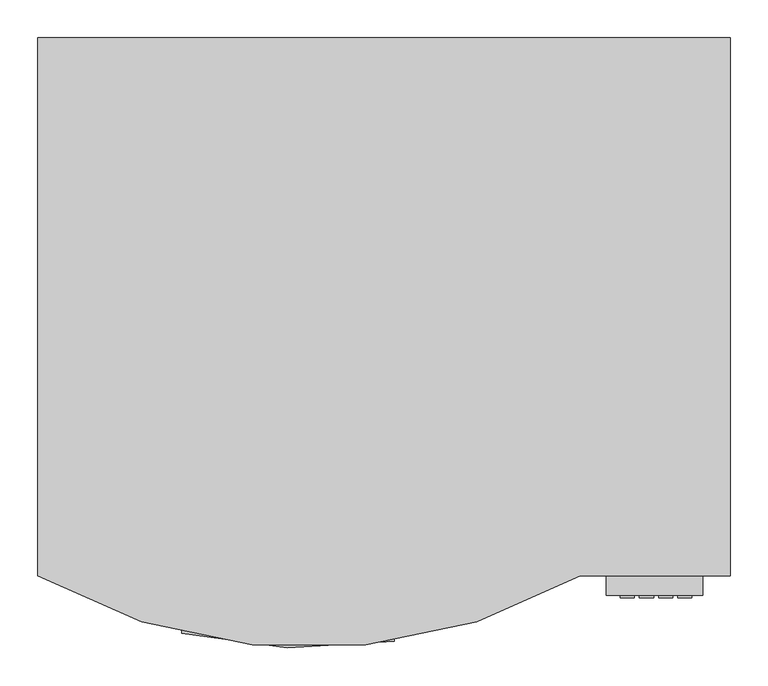
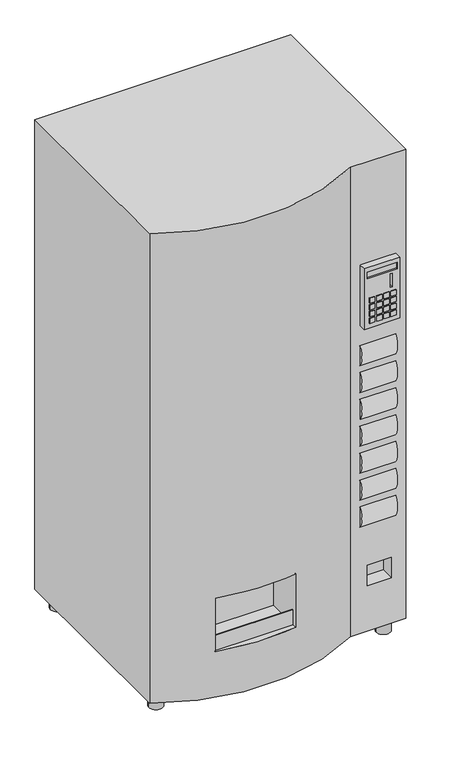
"""IFC4 building model written with IfcOpenShell, lengths in millimetres: proxy geometry, Getränkeautomat : Getränkeautomat."""

from ifc_helpers import new_model, si_unit, point, frame, frame_2d, origin, origin_with_axes, place, context, project, spatial, polyline, circle_curve, trimmed, segment, composite_curve, outline, extrude, faceted_brep, source, transform, mapped, element, save
from ifc_brep_helpers import plane_surface, cylinder_surface, advanced_brep


def specialty_equipment_d6c7ff97(model_context):
    return source(origin(), model_context, "Body", "SolidModel", [
        extrude(outline(composite_curve([segment(trimmed(circle_curve(frame_2d((-216.0902216, 1105.4279487)), 67.5221597), [point((-271.8363609, 1067.3279487))], [point((-271.8363609, 1143.5279487))], False, "CARTESIAN"), True, "CONTINUOUS"), segment(polyline([(-271.8363609, 1143.5279487), (-271.8363609, 1067.3279487)]), True, "CONTINUOUS")], self_intersect=False)), frame((275.3159229, 0.0, 0.0), z_axis=(1.0, 0.0, 0.0), x_axis=(0.0, 1.0, 0.0)), (0.0, 0.0, 1.0), 127.0948963),
        extrude(outline(composite_curve([segment(trimmed(circle_curve(frame_2d((-216.0902216, 1003.8279487)), 67.5221597), [point((-271.8363609, 965.7279487))], [point((-271.8363609, 1041.9279487))], False, "CARTESIAN"), True, "CONTINUOUS"), segment(polyline([(-271.8363609, 1041.9279487), (-271.8363609, 965.7279487)]), True, "CONTINUOUS")], self_intersect=False)), frame((275.3159229, 0.0, 0.0), z_axis=(1.0, 0.0, 0.0), x_axis=(0.0, 1.0, 0.0)), (0.0, 0.0, 1.0), 127.0948963),
        extrude(outline(composite_curve([segment(trimmed(circle_curve(frame_2d((-216.0902216, 902.2279487)), 67.5221597), [point((-271.8363609, 864.1279487))], [point((-271.8363609, 940.3279487))], False, "CARTESIAN"), True, "CONTINUOUS"), segment(polyline([(-271.8363609, 940.3279487), (-271.8363609, 864.1279487)]), True, "CONTINUOUS")], self_intersect=False)), frame((275.3159229, 0.0, 0.0), z_axis=(1.0, 0.0, 0.0), x_axis=(0.0, 1.0, 0.0)), (0.0, 0.0, 1.0), 127.0948963),
        extrude(outline(composite_curve([segment(trimmed(circle_curve(frame_2d((-216.0902216, 800.6279487)), 67.5221597), [point((-271.8363609, 762.5279487))], [point((-271.8363609, 838.7279487))], False, "CARTESIAN"), True, "CONTINUOUS"), segment(polyline([(-271.8363609, 838.7279487), (-271.8363609, 762.5279487)]), True, "CONTINUOUS")], self_intersect=False)), frame((275.3159229, 0.0, 0.0), z_axis=(1.0, 0.0, 0.0), x_axis=(0.0, 1.0, 0.0)), (0.0, 0.0, 1.0), 127.0948963),
        extrude(outline(composite_curve([segment(trimmed(circle_curve(frame_2d((-216.0902216, 699.0279487)), 67.5221597), [point((-271.8363609, 660.9279487))], [point((-271.8363609, 737.1279487))], False, "CARTESIAN"), True, "CONTINUOUS"), segment(polyline([(-271.8363609, 737.1279487), (-271.8363609, 660.9279487)]), True, "CONTINUOUS")], self_intersect=False)), frame((275.3159229, 0.0, 0.0), z_axis=(1.0, 0.0, 0.0), x_axis=(0.0, 1.0, 0.0)), (0.0, 0.0, 1.0), 127.0948963),
        extrude(outline(composite_curve([segment(trimmed(circle_curve(frame_2d((-216.0902216, 597.4279487)), 67.5221597), [point((-271.8363609, 559.3279487))], [point((-271.8363609, 635.5279487))], False, "CARTESIAN"), True, "CONTINUOUS"), segment(polyline([(-271.8363609, 635.5279487), (-271.8363609, 559.3279487)]), True, "CONTINUOUS")], self_intersect=False)), frame((275.3159229, 0.0, 0.0), z_axis=(1.0, 0.0, 0.0), x_axis=(0.0, 1.0, 0.0)), (0.0, 0.0, 1.0), 127.0948963),
        extrude(outline(composite_curve([segment(trimmed(circle_curve(frame_2d((-216.0902216, 495.8279487)), 67.5221597), [point((-271.8363609, 457.7279487))], [point((-271.8363609, 533.9279487))], False, "CARTESIAN"), True, "CONTINUOUS"), segment(polyline([(-271.8363609, 533.9279487), (-271.8363609, 457.7279487)]), True, "CONTINUOUS")], self_intersect=False)), frame((275.3159229, 0.0, 0.0), z_axis=(1.0, 0.0, 0.0), x_axis=(0.0, 1.0, 0.0)), (0.0, 0.0, 1.0), 127.0948963),
        faceted_brep([(402.3159229, -297.2363609, 1448.3279487), (275.3159229, -297.2363609, 1448.3279487), (275.3159229, -297.2363609, 1219.7279487), (402.3159229, -297.2363609, 1219.7279487), (286.3445758, -297.2363609, 1432.5207795), (394.2945758, -297.2363609, 1432.5207795), (394.2945758, -297.2363609, 1407.1207795), (286.3445758, -297.2363609, 1407.1207795), (369.009172, -297.2363609, 1397.7730022), (375.359172, -297.2363609, 1397.7730022), (375.359172, -297.2363609, 1346.9730022), (369.009172, -297.2363609, 1346.9730022), (402.3159229, -271.8363609, 1448.3279487), (402.3159229, -271.8363609, 1219.7279487), (275.3159229, -271.8363609, 1219.7279487), (275.3159229, -271.8363609, 1448.3279487), (394.2945758, -290.8863609, 1432.5207795), (286.3445758, -290.8863609, 1432.5207795), (286.3445758, -290.8863609, 1407.1207795), (394.2945758, -290.8863609, 1407.1207795), (375.359172, -275.0113609, 1397.7730022), (369.009172, -275.0113609, 1397.7730022), (369.009172, -275.0113609, 1346.9730022), (375.359172, -275.0113609, 1346.9730022)], [[[0, 1, 2, 3], [4, 5, 6, 7], [8, 9, 10, 11]], [[12, 13, 14, 15]], [[1, 0, 12, 15]], [[2, 1, 15, 14]], [[3, 2, 14, 13]], [[0, 3, 13, 12]], [[16, 17, 18, 19]], [[17, 16, 5, 4]], [[18, 17, 4, 7]], [[19, 18, 7, 6]], [[16, 19, 6, 5]], [[20, 21, 22, 23]], [[21, 20, 9, 8]], [[22, 21, 8, 11]], [[23, 22, 11, 10]], [[20, 23, 10, 9]]]),
        extrude(outline(polyline([(-4.9505365, -342.4801109), (-285.8560243, -342.4801109), (-285.8560243, -339.3678837), (-4.9505365, -339.3678837), (-4.9505365, -342.4801109)])), frame((0.0, 0.0, 227.0552601), z_axis=(0.0, 0.0, 1.0), x_axis=(1.0, 0.0, 0.0)), (0.0, 0.0, 1.0), 59.7862005),
        extrude(outline(composite_curve([segment(trimmed(circle_curve(frame_2d((-424.8751183, 388.5636391)), 25.4), [point((-450.2751183, 388.5636391))], [point((-399.4751183, 388.5636391))], False, "CARTESIAN"), True, "CONTINUOUS"), segment(trimmed(circle_curve(frame_2d((-424.8751183, 388.5636391)), 25.4), [point((-399.4751183, 388.5636391))], [point((-450.2751183, 388.5636391))], False, "CARTESIAN"), True, "CONTINUOUS")], self_intersect=False)), origin_with_axes(), (0.0, 0.0, 1.0), 55.5625),
        extrude(outline(composite_curve([segment(trimmed(circle_curve(frame_2d((387.9248817, 388.5636391)), 25.4), [point((362.5248817, 388.5636391))], [point((413.3248817, 388.5636391))], False, "CARTESIAN"), True, "CONTINUOUS"), segment(trimmed(circle_curve(frame_2d((387.9248817, 388.5636391)), 25.4), [point((413.3248817, 388.5636391))], [point((362.5248817, 388.5636391))], False, "CARTESIAN"), True, "CONTINUOUS")], self_intersect=False)), origin_with_axes(), (0.0, 0.0, 1.0), 55.5625),
        extrude(outline(composite_curve([segment(trimmed(circle_curve(frame_2d((387.9248817, -221.0363609)), 25.4), [point((362.5248817, -221.0363609))], [point((413.3248817, -221.0363609))], False, "CARTESIAN"), True, "CONTINUOUS"), segment(trimmed(circle_curve(frame_2d((387.9248817, -221.0363609)), 25.4), [point((413.3248817, -221.0363609))], [point((362.5248817, -221.0363609))], False, "CARTESIAN"), True, "CONTINUOUS")], self_intersect=False)), origin_with_axes(), (0.0, 0.0, 1.0), 55.5625),
        extrude(outline(composite_curve([segment(trimmed(circle_curve(frame_2d((-424.8751183, -221.0363609)), 25.4), [point((-450.2751183, -221.0363609))], [point((-399.4751183, -221.0363609))], False, "CARTESIAN"), True, "CONTINUOUS"), segment(trimmed(circle_curve(frame_2d((-424.8751183, -221.0363609)), 25.4), [point((-399.4751183, -221.0363609))], [point((-450.2751183, -221.0363609))], False, "CARTESIAN"), True, "CONTINUOUS")], self_intersect=False)), origin_with_axes(), (0.0, 0.0, 1.0), 55.5625),
        advanced_brep(
        [(438.7248817, 439.3636391, 1828.8), (-475.6751183, 439.3636391, 1828.8), (-475.6751183, -271.8363609, 1828.8), (240.962407, -271.8363609, 1828.8), (438.7248817, -271.8363609, 1828.8), (438.7248817, 439.3636391, 55.4895962), (438.7248817, -271.8363609, 55.4895962), (240.962407, -271.8363609, 55.4895962), (-475.6751183, -271.8363609, 55.4895962), (-475.6751183, 439.3636391, 55.4895962), (-285.8560243, -347.1225541, 431.8), (-4.9505365, -358.2607189, 431.8), (-4.9505365, -358.2607189, 229.9895559), (-285.8560243, -347.1225541, 229.9895559), (387.9248817, -271.8363609, 304.8), (387.9248817, -271.8363609, 227.0552601), (301.300731, -271.8363609, 227.0552601), (301.300731, -271.8363609, 304.8), (-4.9505365, -221.0363609, 431.8), (-285.8560243, -221.0363609, 431.8), (-285.8560243, -221.0363609, 229.9895559), (-4.9505365, -221.0363609, 229.9895559), (387.9248817, -221.0363609, 304.8), (301.300731, -221.0363609, 304.8), (301.300731, -221.0363609, 227.0552601), (387.9248817, -221.0363609, 227.0552601)],
        [
            (0, 1),
            (1, 2),
            (2, 3, circle_curve(frame((-117.3563557, 354.6542517, 1828.8), z_axis=(0.0, 0.0, 1.0), x_axis=(1.0, 0.0, 0.0)), 721.7221234)),
            (3, 4),
            (4, 0),
            (5, 6),
            (6, 7),
            (7, 8, circle_curve(frame((-117.3563557, 354.6542517, 55.4895962), z_axis=(0.0, 0.0, -1.0), x_axis=(1.0, 0.0, 0.0)), 721.7221234)),
            (8, 9),
            (9, 5),
            (0, 5),
            (9, 1),
            (8, 2),
            (7, 3),
            (10, 11, circle_curve(frame((-117.3563557, 354.6542517, 431.8), z_axis=(0.0, 0.0, 1.0), x_axis=(1.0, 0.0, 0.0)), 721.7221234)),
            (11, 12),
            (12, 13, circle_curve(frame((-117.3563557, 354.6542517, 229.9895559), z_axis=(0.0, 0.0, -1.0), x_axis=(1.0, 0.0, 0.0)), 721.7221234)),
            (13, 10),
            (6, 4),
            (14, 15),
            (15, 16),
            (16, 17),
            (17, 14),
            (18, 19),
            (19, 20),
            (20, 21),
            (21, 18),
            (18, 11),
            (10, 19),
            (13, 20),
            (12, 21),
            (22, 23),
            (23, 24),
            (24, 25),
            (25, 22),
            (25, 15),
            (14, 22),
            (24, 16),
            (23, 17),
        ],
        [
            plane_surface(frame((-475.6751183, 439.3636391, 1828.8), z_axis=(0.0, 0.0, 1.0), x_axis=(-1.0, 0.0, 0.0))),
            plane_surface(frame((-475.6751183, 439.3636391, 55.4895962), z_axis=(0.0, 0.0, -1.0), x_axis=(1.0, 0.0, 0.0))),
            plane_surface(frame((438.7248817, 439.3636391, 1828.8), z_axis=(0.0, 1.0, 0.0), x_axis=(0.0, 0.0, -1.0))),
            plane_surface(frame((-475.6751183, 439.3636391, 1828.8), z_axis=(-1.0, 0.0, 0.0), x_axis=(0.0, 0.0, -1.0))),
            cylinder_surface(frame((-117.3563557, 354.6542517, 55.4895962), z_axis=(0.0, 0.0, 1.0), x_axis=(1.0, 0.0, 0.0)), 721.7221234),
            plane_surface(frame((240.962407, -271.8363609, 1828.8), z_axis=(0.0, -1.0, 0.0), x_axis=(0.0, 0.0, -1.0))),
            plane_surface(frame((438.7248817, -271.8363609, 1828.8), z_axis=(1.0, 0.0, 0.0), x_axis=(0.0, 0.0, -1.0))),
            plane_surface(frame((-285.8560243, -221.0363609, 431.8), z_axis=(0.0, -1.0, 0.0), x_axis=(1.0, 0.0, 0.0))),
            plane_surface(frame((-4.9505365, -383.6604873, 431.8), z_axis=(0.0, 0.0, -1.0), x_axis=(0.0, 1.0, 0.0))),
            plane_surface(frame((-285.8560243, -383.6604873, 431.8), z_axis=(1.0, 0.0, 0.0), x_axis=(0.0, 1.0, 0.0))),
            plane_surface(frame((-285.8560243, -383.6604873, 229.9895559), z_axis=(0.0, 0.0, 1.0), x_axis=(0.0, 1.0, 0.0))),
            plane_surface(frame((-4.9505365, -383.6604873, 229.9895559), z_axis=(-1.0, 0.0, 0.0), x_axis=(0.0, 1.0, 0.0))),
            plane_surface(frame((387.9248817, -221.0363609, 304.8), z_axis=(0.0, -1.0, 0.0), x_axis=(0.0, 0.0, -1.0))),
            plane_surface(frame((387.9248817, -221.0363609, 304.8), z_axis=(-1.0, 0.0, 0.0), x_axis=(0.0, -1.0, 0.0))),
            plane_surface(frame((387.9248817, -221.0363609, 227.0552601), z_axis=(0.0, 0.0, 1.0), x_axis=(0.0, -1.0, 0.0))),
            plane_surface(frame((301.300731, -221.0363609, 227.0552601), z_axis=(1.0, 0.0, 0.0), x_axis=(0.0, -1.0, 0.0))),
            plane_surface(frame((301.300731, -221.0363609, 304.8), z_axis=(0.0, 0.0, -1.0), x_axis=(0.0, -1.0, 0.0))),
        ],
        [
            (0, [[1, 2, 3, 4, 5]]),
            (1, [[6, 7, 8, 9, 10]]),
            (2, [[-1, 11, -10, 12]]),
            (3, [[-2, -12, -9, 13]]),
            (4, [[-3, -13, -8, 14], [15, 16, 17, 18]]),
            (5, [[-4, -14, -7, 19], [20, 21, 22, 23]]),
            (6, [[-5, -19, -6, -11]]),
            (7, [[24, 25, 26, 27]]),
            (8, [[-24, 28, -15, 29]]),
            (9, [[-25, -29, -18, 30]]),
            (10, [[-26, -30, -17, 31]]),
            (11, [[-27, -31, -16, -28]]),
            (12, [[32, 33, 34, 35]]),
            (13, [[-35, 36, -20, 37]]),
            (14, [[-34, 38, -21, -36]]),
            (15, [[-33, 39, -22, -38]]),
            (16, [[-32, -37, -23, -39]]),
        ],
    ),
        extrude(outline(polyline([(312.3802372, -300.4113609), (293.3302372, -300.4113609), (293.3302372, -297.2363609), (312.3802372, -297.2363609), (312.3802372, -300.4113609)])), frame((0.0, 0.0, 1313.6452473), z_axis=(0.0, 0.0, 1.0), x_axis=(1.0, 0.0, 0.0)), (0.0, 0.0, 1.0), 19.05),
        extrude(outline(polyline([(312.3802372, -300.4113609), (293.3302372, -300.4113609), (293.3302372, -297.2363609), (312.3802372, -297.2363609), (312.3802372, -300.4113609)])), frame((0.0, 0.0, 1237.4452473), z_axis=(0.0, 0.0, 1.0), x_axis=(1.0, 0.0, 0.0)), (0.0, 0.0, 1.0), 19.05),
        extrude(outline(polyline([(387.9248817, -300.4113609), (369.5302372, -300.4113609), (369.5302372, -297.2363609), (387.9248817, -297.2363609), (387.9248817, -300.4113609)])), frame((0.0, 0.0, 1237.4452473), z_axis=(0.0, 0.0, 1.0), x_axis=(1.0, 0.0, 0.0)), (0.0, 0.0, 1.0), 19.05),
        extrude(outline(polyline([(387.9248817, -300.4113609), (369.5302372, -300.4113609), (369.5302372, -297.2363609), (387.9248817, -297.2363609), (387.9248817, -300.4113609)])), frame((0.0, 0.0, 1313.6452473), z_axis=(0.0, 0.0, 1.0), x_axis=(1.0, 0.0, 0.0)), (0.0, 0.0, 1.0), 19.05),
        extrude(outline(polyline([(312.3802372, -300.4113609), (293.3302372, -300.4113609), (293.3302372, -297.2363609), (312.3802372, -297.2363609), (312.3802372, -300.4113609)])), frame((0.0, 0.0, 1288.2452473), z_axis=(0.0, 0.0, 1.0), x_axis=(1.0, 0.0, 0.0)), (0.0, 0.0, 1.0), 19.05),
        extrude(outline(polyline([(312.3802372, -300.4113609), (293.3302372, -300.4113609), (293.3302372, -297.2363609), (312.3802372, -297.2363609), (312.3802372, -300.4113609)])), frame((0.0, 0.0, 1262.8452473), z_axis=(0.0, 0.0, 1.0), x_axis=(1.0, 0.0, 0.0)), (0.0, 0.0, 1.0), 19.05),
        extrude(outline(polyline([(337.7802372, -300.4113609), (318.7302372, -300.4113609), (318.7302372, -297.2363609), (337.7802372, -297.2363609), (337.7802372, -300.4113609)])), frame((0.0, 0.0, 1313.6452473), z_axis=(0.0, 0.0, 1.0), x_axis=(1.0, 0.0, 0.0)), (0.0, 0.0, 1.0), 19.05),
        extrude(outline(polyline([(363.1802372, -300.4113609), (344.1302372, -300.4113609), (344.1302372, -297.2363609), (363.1802372, -297.2363609), (363.1802372, -300.4113609)])), frame((0.0, 0.0, 1313.6452473), z_axis=(0.0, 0.0, 1.0), x_axis=(1.0, 0.0, 0.0)), (0.0, 0.0, 1.0), 19.05),
        extrude(outline(polyline([(337.7802372, -300.4113609), (318.7302372, -300.4113609), (318.7302372, -297.2363609), (337.7802372, -297.2363609), (337.7802372, -300.4113609)])), frame((0.0, 0.0, 1237.4452473), z_axis=(0.0, 0.0, 1.0), x_axis=(1.0, 0.0, 0.0)), (0.0, 0.0, 1.0), 19.05),
        extrude(outline(polyline([(363.1802372, -300.4113609), (344.1302372, -300.4113609), (344.1302372, -297.2363609), (363.1802372, -297.2363609), (363.1802372, -300.4113609)])), frame((0.0, 0.0, 1237.4452473), z_axis=(0.0, 0.0, 1.0), x_axis=(1.0, 0.0, 0.0)), (0.0, 0.0, 1.0), 19.05),
        extrude(outline(polyline([(387.9248817, -300.4113609), (369.5302372, -300.4113609), (369.5302372, -297.2363609), (387.9248817, -297.2363609), (387.9248817, -300.4113609)])), frame((0.0, 0.0, 1262.8452473), z_axis=(0.0, 0.0, 1.0), x_axis=(1.0, 0.0, 0.0)), (0.0, 0.0, 1.0), 19.05),
        extrude(outline(polyline([(387.9248817, -300.4113609), (369.5302372, -300.4113609), (369.5302372, -297.2363609), (387.9248817, -297.2363609), (387.9248817, -300.4113609)])), frame((0.0, 0.0, 1288.2452473), z_axis=(0.0, 0.0, 1.0), x_axis=(1.0, 0.0, 0.0)), (0.0, 0.0, 1.0), 19.05),
        extrude(outline(polyline([(337.7802372, -300.4113609), (318.7302372, -300.4113609), (318.7302372, -297.2363609), (337.7802372, -297.2363609), (337.7802372, -300.4113609)])), frame((0.0, 0.0, 1262.8452473), z_axis=(0.0, 0.0, 1.0), x_axis=(1.0, 0.0, 0.0)), (0.0, 0.0, 1.0), 19.05),
        extrude(outline(polyline([(363.1802372, -300.4113609), (344.1302372, -300.4113609), (344.1302372, -297.2363609), (363.1802372, -297.2363609), (363.1802372, -300.4113609)])), frame((0.0, 0.0, 1262.8452473), z_axis=(0.0, 0.0, 1.0), x_axis=(1.0, 0.0, 0.0)), (0.0, 0.0, 1.0), 19.05),
        extrude(outline(polyline([(363.1802372, -300.4113609), (344.1302372, -300.4113609), (344.1302372, -297.2363609), (363.1802372, -297.2363609), (363.1802372, -300.4113609)])), frame((0.0, 0.0, 1288.2452473), z_axis=(0.0, 0.0, 1.0), x_axis=(1.0, 0.0, 0.0)), (0.0, 0.0, 1.0), 19.05),
        extrude(outline(polyline([(337.7802372, -300.4113609), (318.7302372, -300.4113609), (318.7302372, -297.2363609), (337.7802372, -297.2363609), (337.7802372, -300.4113609)])), frame((0.0, 0.0, 1288.2452473), z_axis=(0.0, 0.0, 1.0), x_axis=(1.0, 0.0, 0.0)), (0.0, 0.0, 1.0), 19.05),
    ])


if __name__ == "__main__":
    model = new_model("IFC4")
    model_context = context("Model", 3, world=origin())
    ifc_project = project(units=[si_unit("LENGTHUNIT", "METRE", prefix="MILLI")], contexts=[model_context])
    site = spatial("IfcSite", under=ifc_project)
    building = spatial("IfcBuilding", under=site)
    placement = place(None, origin())
    specialty_equipment_shape = specialty_equipment_d6c7ff97(model_context)
    element("IfcBuildingElementProxy", 1, Name="Getränkeautomat : Getränkeautomat", ObjectType="Getränkeautomat : Getränkeautomat", at=placement, inside=building, context=model_context, shape_type="MappedRepresentation", body=[
        mapped(specialty_equipment_shape, transform((0.0, 0.0, 0.0), x_axis=(1.0, 0.0, 0.0), y_axis=(0.0, 1.0, 0.0), z_axis=(0.0, 0.0, 1.0))),
    ])
    save(model, "model.ifc")

# Revit data of these elements
# Type "Getränkeautomat : Getränkeautomat"
#   Assembly Code = ""
# Element 1 (IfcBuildingElementProxy, "Getränkeautomat : Getränkeautomat")
#   Materials on its faces: "Metall - Edelstahl", "Kunststoff - Braun", "Metall - Stahl"
# Materials
#   "Metall - Edelstahl": class "Metall", colour RGB 176 176 176, transparency 0
#   "Kunststoff - Braun": class "Kunststoff", colour RGB 176 109 71, transparency 0
#   "Metall - Stahl": class "Metall", colour RGB 247 247 247, transparency 0, Cost = 0
